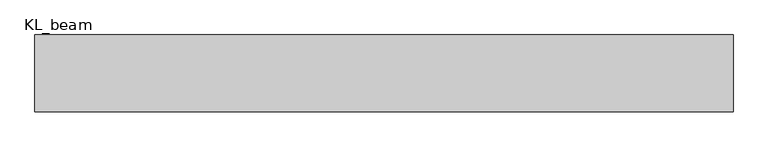
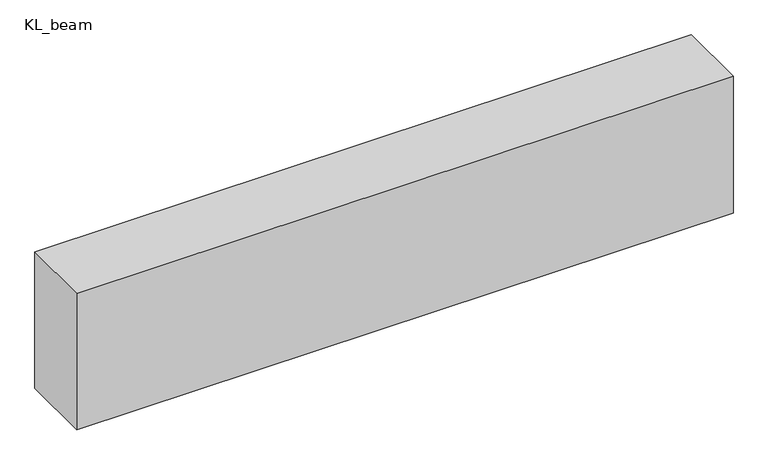
"""IFC4 building model written with IfcOpenShell, lengths in millimetres: beam geometry, 混凝土 - 矩形梁 : KL_beam."""

from ifc_helpers import new_model, si_unit, frame, origin, place, context, project, spatial, polyline, outline, extrude, source, transform, mapped, element, save


def kl_beam_c459b6d2(model_context):
    return source(origin(), model_context, "Body", "SweptSolid", [
        extrude(outline(polyline([(1817.0, 200.0), (1817.0, -200.0), (-1817.0, -200.0), (-1817.0, 200.0), (1817.0, 200.0)])), frame((0.0, 0.0, -400.0), z_axis=(0.0, 0.0, 1.0), x_axis=(1.0, 0.0, 0.0)), (0.0, 0.0, 1.0), 800.0),
    ])


if __name__ == "__main__":
    model = new_model("IFC4")
    model_context = context("Model", 3, world=origin())
    ifc_project = project(units=[si_unit("LENGTHUNIT", "METRE", prefix="MILLI")], contexts=[model_context])
    site = spatial("IfcSite", under=ifc_project)
    building = spatial("IfcBuilding", under=site)
    placement = place(None, origin())
    kl_beam_shape = kl_beam_c459b6d2(model_context)
    element("IfcBeam", 1, ObjectType="混凝土 - 矩形梁 : KL_beam", at=placement, inside=building, context=model_context, shape_type="MappedRepresentation", body=[
        mapped(kl_beam_shape, transform((0.0, 0.0, 0.0), x_axis=(1.0, 0.0, 0.0), y_axis=(0.0, 1.0, 0.0), z_axis=(0.0, 0.0, 1.0))),
    ])
    save(model, "model.ifc")

# Revit data of these elements
# Type "混凝土 - 矩形梁 : KL_beam"
#   Length [instance default] = 1524 mm
#   b = 400 mm
#   h = 800 mm
#   Structural Material [instance default] = 混凝土 - 现场浇注混凝土
#   Assembly Code = ""
# Element 1 (IfcBeam, "混凝土 - 矩形梁 : KL_beam")
#   Structural Material = none
# Materials
#   "混凝土 - 现场浇注混凝土": class "混凝土", colour RGB 192 192 192, transparency 0
